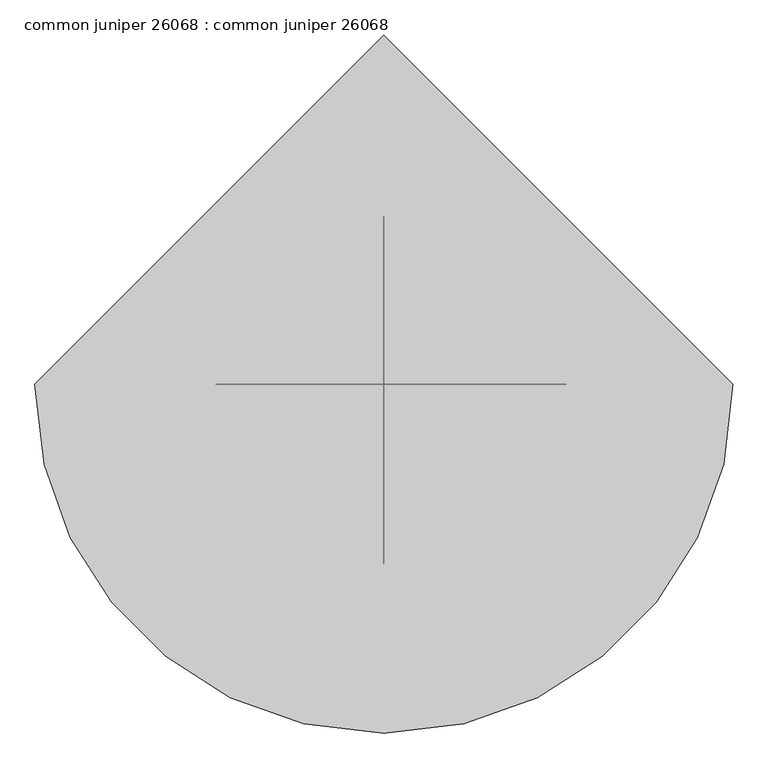
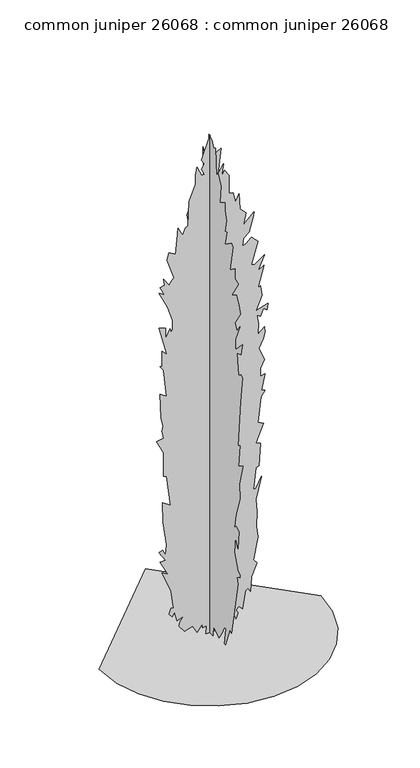
"""IFC4 building model written with IfcOpenShell, lengths in millimetres: proxy geometry, common juniper 26068 : common juniper 26068."""

import ifcopenshell
import ifcopenshell.guid

model = None  # the IFC model being written
_history = None  # IfcOwnerHistory: only IFC2X3 demands one
_inside = {}  # id of a spatial element -> (the spatial element, [elements in it])
_under = {}  # id of a project, library or spatial element -> (it, [spatial elements below it])
_declared = {}  # id of a project -> (the project, [libraries it declares])
_typed = {}  # id of a type object -> (the type object, [elements of that type])
_made_of = {}  # id of a material, layer set ... -> (it, [elements and type objects made of it])


def new_model(schema):
    """Start an empty IFC model of exactly this schema.

    Asked for "IFC4X3", IfcOpenShell would pick the latest addendum, in which some entities
    have other attributes; the version numbers below select the first issue.
    IFC2X3 requires an IfcOwnerHistory on every rooted entity: one is made here for all.
    """
    global model, _history
    if schema == "IFC4X3":
        model = ifcopenshell.file(schema_version=(4, 3, 0, 0))
    else:
        model = ifcopenshell.file(schema=schema)
    _inside.clear()
    _under.clear()
    _declared.clear()
    _typed.clear()
    _made_of.clear()
    _history = None
    if model.schema == "IFC2X3":
        org = make("IfcOrganization", Name="unknown")
        user = make(
            "IfcPersonAndOrganization",
            ThePerson=make("IfcPerson", FamilyName="unknown"),
            TheOrganization=org,
        )
        app = make(
            "IfcApplication",
            ApplicationDeveloper=org,
            Version="unknown",
            ApplicationFullName="unknown",
            ApplicationIdentifier="unknown",
        )
        _history = make(
            "IfcOwnerHistory",
            OwningUser=user,
            OwningApplication=app,
            ChangeAction="ADDED",
            CreationDate=0,
        )
    return model


def make(cls, **values):
    """One entity of the class cls with the attributes given. An attribute that is None is left unset."""
    return model.create_entity(
        cls, **{name: value for name, value in values.items() if value is not None}
    )


def rooted(cls, **values):
    """An entity with a GlobalId (a new one), such as an element, a storey or a relation."""
    return make(cls, GlobalId=ifcopenshell.guid.new(), OwnerHistory=_history, **values)


def si_unit(unit_type, name, prefix=None):
    """IfcSIUnit, for example si_unit("LENGTHUNIT", "METRE", prefix="MILLI")."""
    return make("IfcSIUnit", UnitType=unit_type, Prefix=prefix, Name=name)


def assignment(units):
    """IfcUnitAssignment: the units of a project."""
    return None if units is None else make("IfcUnitAssignment", Units=units)


def point(xyz):
    """IfcCartesianPoint."""
    return None if xyz is None else make("IfcCartesianPoint", Coordinates=xyz)


def direction(xyz):
    """IfcDirection."""
    return None if xyz is None else make("IfcDirection", DirectionRatios=xyz)


def frame(location, z_axis=None, x_axis=None):
    """IfcAxis2Placement3D, a coordinate frame: its origin and axes. An axis left out is left unset."""
    return make(
        "IfcAxis2Placement3D",
        Location=point(location),
        Axis=direction(z_axis),
        RefDirection=direction(x_axis),
    )


def origin():
    """The frame at (0, 0, 0) with its axes left unset."""
    return frame((0.0, 0.0, 0.0))


def place(relative_to, where):
    """IfcLocalPlacement: puts the frame where relative to a parent placement (None: the world)."""
    return make(
        "IfcLocalPlacement", PlacementRelTo=relative_to, RelativePlacement=where
    )


def context(
    kind, dimensions, precision=None, world=None, true_north=None, identifier=None
):
    """IfcGeometricRepresentationContext, for example the 3D "Model" context."""
    return make(
        "IfcGeometricRepresentationContext",
        ContextIdentifier=identifier,
        ContextType=kind,
        CoordinateSpaceDimension=dimensions,
        Precision=precision,
        WorldCoordinateSystem=world,
        TrueNorth=true_north,
    )


def project(units=None, contexts=None):
    """IfcProject with its units and contexts."""
    return rooted(
        "IfcProject",
        Name="project",
        RepresentationContexts=contexts,
        UnitsInContext=assignment(units),
    )


def spatial(cls, under=None, at=None, **own):
    """A site, building, storey or space (cls), placed at a placement, below another one or the project."""
    s = rooted(cls, ObjectPlacement=at, **own)
    if under is not None:
        _under.setdefault(under.id(), (under, []))[1].append(s)
    return s


def point_list(points):
    """IfcCartesianPointList2D or 3D."""
    cls = (
        "IfcCartesianPointList2D" if len(points[0]) == 2 else "IfcCartesianPointList3D"
    )
    return make(cls, CoordList=points)


def triangles(points, corners, closed=None, point_numbers=None):
    """IfcTriangulatedFaceSet: each triangle names its three corners, points numbered from 1."""
    return make(
        "IfcTriangulatedFaceSet",
        Coordinates=point_list(points),
        Closed=closed,
        CoordIndex=corners,
        PnIndex=point_numbers,
    )


def shape(context_of_items, identifier, shape_type, items):
    """IfcShapeRepresentation: the items that make up one representation, for example the "Body"."""
    return make(
        "IfcShapeRepresentation",
        ContextOfItems=context_of_items,
        RepresentationIdentifier=identifier,
        RepresentationType=shape_type,
        Items=items,
    )


def source(mapping_origin, context_of_items, identifier, shape_type, items):
    """IfcRepresentationMap: a shape defined once, which mapped items show again and again."""
    return make(
        "IfcRepresentationMap",
        MappingOrigin=mapping_origin,
        MappedRepresentation=shape(context_of_items, identifier, shape_type, items),
    )


def transform(
    local_origin,
    x_axis=None,
    y_axis=None,
    z_axis=None,
    scale=None,
    scale2=None,
    scale3=None,
    uniform=True,
):
    """IfcCartesianTransformationOperator3D, or its non-uniform kind. x_axis, y_axis, z_axis: its Axis1, 2, 3."""
    if uniform:
        return make(
            "IfcCartesianTransformationOperator3D",
            Axis1=direction(x_axis),
            Axis2=direction(y_axis),
            LocalOrigin=point(local_origin),
            Scale=scale,
            Axis3=direction(z_axis),
        )
    return make(
        "IfcCartesianTransformationOperator3DnonUniform",
        Axis1=direction(x_axis),
        Axis2=direction(y_axis),
        LocalOrigin=point(local_origin),
        Scale=scale,
        Axis3=direction(z_axis),
        Scale2=scale2,
        Scale3=scale3,
    )


def mapped(mapping_source, mapping_target):
    """IfcMappedItem: shows the shape of a source again, moved by a transform."""
    return make(
        "IfcMappedItem", MappingSource=mapping_source, MappingTarget=mapping_target
    )


def made_of(thing, what):
    """Note that an element or type object is made of a material, layer set ...; save() writes the relation."""
    if what is not None:
        _made_of.setdefault(what.id(), (what, []))[1].append(thing)
    return thing


def element(
    cls,
    number,
    at=None,
    inside=None,
    cuts=None,
    type_object=None,
    material=None,
    context=None,
    identifier="Body",
    shape_type=None,
    held_by="IfcProductDefinitionShape",
    body=None,
    shapes=None,
    **own,
):
    """One element of the class cls, such as IfcWall. Its Tag is "e" and its number.

    at: its placement. inside: the storey or other place that contains it. cuts: it is an
    opening in that element (IfcRelVoidsElement). A single representation is given by context,
    identifier, shape_type and body (its items); several are given by shapes. held_by: the class
    of the entity that holds the representations. save() writes the other relations.
    """
    e = rooted(cls, Tag="e%d" % number, ObjectPlacement=at, **own)
    if body is not None:
        shapes = [shape(context, identifier, shape_type, body)]
    if shapes is not None:
        e.Representation = make(held_by, Representations=shapes)
    if inside is not None:
        _inside.setdefault(inside.id(), (inside, []))[1].append(e)
    if cuts is not None:
        rooted(
            "IfcRelVoidsElement", RelatingBuildingElement=cuts, RelatedOpeningElement=e
        )
    if type_object is not None:
        _typed.setdefault(type_object.id(), (type_object, []))[1].append(e)
    return made_of(e, material)


def aggregate(whole, parts):
    """IfcRelAggregates: a whole, such as a stair, and the parts it consists of."""
    return rooted("IfcRelAggregates", RelatingObject=whole, RelatedObjects=parts)


def save(model, path):
    """Write the relations noted so far, then the file.

    IfcRelAggregates (storeys below a building ...), IfcRelContainedInSpatialStructure (elements
    in a storey), IfcRelDefinesByType, IfcRelAssociatesMaterial and IfcRelDeclares: one each for
    every whole, place, type object, material and project.
    """
    for whole, parts in _under.values():
        aggregate(whole, parts)
    for where, things in _inside.values():
        rooted(
            "IfcRelContainedInSpatialStructure",
            RelatedElements=things,
            RelatingStructure=where,
        )
    for kind, things in _typed.values():
        rooted("IfcRelDefinesByType", RelatedObjects=things, RelatingType=kind)
    for what, things in _made_of.values():
        rooted("IfcRelAssociatesMaterial", RelatedObjects=things, RelatingMaterial=what)
    for by, libraries in _declared.values():
        rooted("IfcRelDeclares", RelatingContext=by, RelatedDefinitions=libraries)
    model.write(path)


def common_juniper_26068_common_juniper_26068_35e030ca(model_context):
    return source(origin(), model_context, "Body", "Tessellation", [
        triangles([(2e-06, 20.8572502, 34.4973742), (2.9e-06, 50.3272151, 21.867388), (4.9e-06, 67.1674663, 63.9673119), (4e-06, 75.5873421, 21.867388), (6e-06, 105.0572775, 42.9175021), (6.8e-06, 126.1073371, 38.7074393), (1.05e-05, 163.9974026, 106.0674356), (1.16e-05, 163.9974026, 143.9575011), (1.1e-05, 147.1574058, 148.1673096), (1.26e-05, 147.1574058, 202.8973719), (1.29e-05, 176.6273366, 169.2173783), (1.44e-05, 185.0474622, 207.1074347), (1.33e-05, 155.577277, 211.3174975), (1.5e-05, 155.577277, 270.2568686), (1.59e-05, 172.4172738, 274.4682032), (2.15e-05, 208.9710382, 408.6238226), (2.29e-05, 206.0972674, 459.7084588), (2.67e-05, 248.1971505, 522.8581289), (2.46e-05, 201.8872046, 522.8581289), (2.34e-05, 185.1554134, 508.0702234), (2.48e-05, 172.4172738, 573.376339), (2.87e-05, 210.3073302, 649.1574692), (2.78e-05, 174.6776373, 670.1633818), (3.35e-05, 214.5174112, 800.7172588), (3.23e-05, 197.6771419, 788.0883059), (3.52e-05, 206.0972674, 872.2870182), (4.35e-05, 239.7772792, 1099.6279381), (4.31e-05, 214.5174112, 1124.8883148), (4.64e-05, 221.6324747, 1223.064735), (4.69e-05, 206.0972674, 1263.816608), (5.28e-05, 239.7772792, 1411.1674976), (5.42e-05, 214.5174112, 1495.3662827), (5.6e-05, 239.7772792, 1520.6266594), (5.93e-05, 214.5174112, 1667.977549), (5.58e-05, 162.8142626, 1629.2094212), (5.8e-05, 189.2572706, 1663.7663235), (6.33e-05, 189.2572706, 1840.5863445), (6.26e-05, 176.6273366, 1836.3775898), (6.33e-05, 176.6273366, 1857.4265957), (6.27e-05, 163.9971482, 1857.4265957), (6.42e-05, 172.4172738, 1895.3184689), (6.36e-05, 159.7870854, 1895.3184689), (6.46e-05, 172.4172738, 1907.9474945), (6.6e-05, 184.4045872, 1938.4732475), (6.63e-05, 168.207211, 1971.0971283), (6.38e-05, 138.7372802, 1933.2078712), (6.66e-05, 147.1571514, 2013.1977562), (6.57e-05, 130.3171455, 2008.9863853), (6.57e-05, 113.4776574, 2034.2467621), (6.82e-05, 130.3171455, 2093.1876411), (6.79e-05, 117.6872115, 2101.6077667), (6.74e-05, 115.2719156, 2088.51656), (6.69e-05, 112.8578914, 2076.3093109), (6.65e-05, 110.4461564, 2065.872448), (6.62e-05, 108.0382274, 2058.0897835), (6.59e-05, 105.6348767, 2053.8454205), (6.58e-05, 103.2373577, 2054.0233166), (6.59e-05, 100.8472147, 2059.5071388), (6.74e-05, 67.167212, 2160.5486458), (6.91e-05, 79.797146, 2198.4380482), (6.81e-05, 50.3272151, 2211.0669285), (7.25e-05, 54.7259973, 2350.8028759), (6.92e-05, 29.2771487, 2278.4279331), (6.92e-05, 12.4371758, 2303.6883099), (7e-05, 12.4371758, 2328.9486866), (7.13e-05, 1.9569493, 2388.087664), (7.3e-05, 8.22762, 2438.4078484), (7.15e-05, -17.0328629, 2425.7763519), (7.01e-05, -29.662722, 2396.3072205), (6.96e-05, -46.5027211, 2404.727346), (6.53e-05, -54.9228512, 2274.2165623), (6.54e-05, -63.3427225, 2291.0568134), (6.29e-05, -89.9589621, 2244.0082317), (6.07e-05, -82.3490978, 2159.977169), (5.96e-05, -122.2828521, 2181.597797), (5.84e-05, -122.3656505, 2144.5212811), (5.66e-05, -134.9127861, 2101.6077667), (5.54e-05, -122.2828521, 2042.6668877), (5.48e-05, -138.0380133, 2047.4395615), (5.35e-05, -122.2828521, 1979.5172539), (5.23e-05, -172.8028426, 2013.1977562), (5.13e-05, -186.3878237, 2001.8109512), (4.87e-05, -163.5081882, 1878.2927639), (4.78e-05, -202.2725372, 1907.9474945), (4.63e-05, -202.2725372, 1857.4265957), (4.47e-05, -231.7427224, 1849.0064701), (4.47e-05, -177.0129054, 1764.8078304), (4.36e-05, -214.9027256, 1785.8568363), (4.15e-05, -235.9527852, 1747.9675793), (4e-05, -244.3729108, 1710.0783222), (3.99e-05, -202.2725372, 1642.7171722), (3.83e-05, -219.1127884, 1613.2480408), (3.83e-05, -241.2687761, 1646.3393349), (3.74e-05, -205.5590554, 1563.0676735), (3.58e-05, -206.4828544, 1512.2065338), (3.51e-05, -261.2118902, 1571.1474129), (3.4e-05, -248.5827192, 1512.2065338), (3.5e-05, -219.1127884, 1503.7864082), (3.14e-05, -231.7427224, 1402.7473721), (3.11e-05, -248.5827192, 1415.3763977), (3.03e-05, -261.2118902, 1406.9562721), (2.72e-05, -244.3729108, 1280.6568592), (2.12e-05, -227.5326596, 1053.3184828), (2.09e-05, -240.1625937, 1061.7386084), (1.81e-05, -231.7427224, 956.4883467), (1.73e-05, -265.4232247, 977.5373526), (1.54e-05, -237.9499925, 875.0023321), (1.31e-05, -240.1625937, 800.7172588), (1.16e-05, -210.6926628, 703.8870501), (1.01e-05, -198.0627288, 636.5285889), (9.9e-06, -210.6926628, 649.1574692), (8.4e-06, -235.9527852, 636.5285889), (6.2e-06, -227.5326596, 548.1185057), (8.5e-06, -206.4828544, 594.4279246), (6.5e-06, -198.0627288, 514.4380033), (2.9e-06, -227.5326596, 438.6568731), (2e-06, -243.3599639, 431.2197181), (1.5e-06, -243.5103181, 416.411465), (2.3e-06, -219.1127884, 404.9763708), (1e-06, -227.5326596, 375.5071667), (-4.7e-06, -172.8028426, 101.8573729), (-3.9e-06, -160.1726542, 110.2774984), (-5.1e-06, -126.4926606, 17.6574001), (-4.8e-06, -118.0727893, 17.6574001), (-2.9e-06, -130.7027234, 97.6473101), (-2.4e-06, -118.0727893, 97.6473101), (-2.7e-06, -97.022212, 55.5474361), (-2.7e-06, -71.7625937, 17.6574001), (1e-07, -29.662722, 47.1273105), (-1.2e-06, -26.985301, 2.08e-05), (1.1e-06, 25.0673653, 2.23e-05), (-515.3041569, -1e-07, 3.69e-05), (-501.6820959, -118.0735524, 3.3e-05), (-462.8834467, -226.5052332, 2.86e-05), (-402.0172491, -322.1873471, 2.4e-05), (-322.1873471, -402.0172491, 1.92e-05), (-226.5052332, -462.8834467, 1.45e-05), (-118.0735524, -501.6820959, 1.02e-05), (2.25e-05, -515.3041569, 6.2e-06), (118.0735524, -501.6820959, 3.1e-06), (226.5052332, -462.8834467, 1e-06), (322.1873471, -402.0172491, 0.0), (402.0172491, -322.1873471, 0.0), (462.8834467, -226.5052332, 1e-06), (501.6820959, -118.0735524, 3.1e-06), (515.3041569, 4.49e-05, 6.2e-06), (-6.76e-05, 515.3041569, 3.69e-05), (-18.1277839, 9e-07, 2.21e-05), (-15.9294828, -9e-07, 38.9106382), (-33.6886368, -1e-07, 34.4973742), (-33.6886368, -1.1e-06, 55.5474361), (-58.9485094, 1.2e-06, 21.8674629), (-79.998569, 1e-07, 59.7575034), (-117.8886345, 2.9e-06, 47.1273105), (-143.1485116, 2.2e-06, 80.8073133), (-138.9386941, 0.0, 101.8573729), (-122.098443, -1.5e-06, 122.9074415), (-151.5686372, 0.0, 110.2774984), (-164.1985713, -1.7e-06, 156.5874443), (-176.8285053, -6e-07, 139.7474384), (-189.4584393, -1e-06, 156.5874443), (-181.0385681, -2.3e-06, 181.8473123), (-168.4083797, -2.7e-06, 181.8473123), (-180.3558154, -7.3e-06, 266.0887183), (-223.1384511, -1.18e-05, 371.2983756), (-193.6685021, -1.19e-05, 354.4581244), (-231.5585767, -1.51e-05, 426.0279565), (-206.2984361, -1.59e-05, 426.0279565), (-236.2903554, -1.71e-05, 473.5007129), (-218.928897, -1.91e-05, 480.757501), (-206.2984361, -1.81e-05, 451.2883332), (-202.0883733, -2.05e-05, 501.8065433), (-216.5369645, -2.75e-05, 615.9519379), (-218.928897, -3.28e-05, 712.3071756), (-183.4688521, -3.28e-05, 688.38538), (-202.0883733, -4.12e-05, 838.6065159), (-214.7185799, -4.1e-05, 842.8178867), (-214.7185799, -4.73e-05, 956.4883467), (-248.3983191, -5.04e-05, 1023.8468079), (-214.7185799, -5.16e-05, 1028.058106), (-221.9263521, -5.3e-05, 1065.2057659), (-216.8864708, -5.54e-05, 1088.911659), (-227.3485139, -5.7e-05, 1133.3084404), (-231.5585767, -6.44e-05, 1251.1877277), (-202.0883733, -6.44e-05, 1230.1385765), (-214.7185799, -7.1e-05, 1360.6467442), (-231.5585767, -7.27e-05, 1385.9071209), (-223.1384511, -7.28e-05, 1381.6983662), (-223.1384511, -7.73e-05, 1457.4770256), (-199.0627223, -7.69e-05, 1431.8229229), (-235.7683851, -8.33e-05, 1575.3561676), (-205.5140908, -8.37e-05, 1563.9058491), (-206.2984361, -8.14e-05, 1512.2065338), (-185.2483765, -8.39e-05, 1554.3071617), (-181.0385681, -8.33e-05, 1537.4669106), (-172.6184425, -8.39e-05, 1545.8870361), (-172.4459785, -8.71e-05, 1592.2497585), (-195.9021957, -9.07e-05, 1663.7815842), (-235.7683851, -9.33e-05, 1747.9675793), (-210.5084989, -9.33e-05, 1731.1273281), (-231.5585767, -9.57e-05, 1773.227956), (-210.5084989, -9.65e-05, 1777.4367107), (-214.7185799, -9.77e-05, 1806.9084583), (-189.4584393, -9.68e-05, 1769.0165852), (-176.8285053, -9.92e-05, 1790.0682072), (-165.3669774, -9.99e-05, 1797.7949158), (-197.8783105, -0.0001044, 1895.3184689), (-189.4584393, -0.0001062, 1928.9965004), (-159.9885085, -0.0001063, 1912.1562492), (-151.5683829, -0.0001107, 1979.5172539), (-147.3585744, -0.0001144, 2034.2467621), (-126.3085057, -0.0001131, 1992.1461342), (-113.6788261, -0.000115, 2025.8266365), (-101.0483834, -0.0001167, 2030.0380074), (-96.8383206, -0.0001232, 2147.9172947), (-67.4105474, -0.0001297, 2222.3166779), (-67.3683806, -0.0001316, 2265.7964367), (-58.9482551, -0.0001347, 2303.6883099), (-37.8984453, -0.0001321, 2257.3763111), (-25.268484, -0.0001336, 2257.3763111), (-37.8984453, -0.0001346, 2286.8480587), (-25.268484, -0.0001359, 2307.8970646), (-37.8984453, -0.0001365, 2328.9462158), (-0.0084209, -0.0001447, 2438.4078484), (4.2015544, -0.0001387, 2324.7373158), (21.0416299, -0.0001399, 2341.5775669), (33.6716184, -0.0001405, 2345.786467), (50.5116198, -0.0001427, 2358.4178181), (37.8816812, -0.0001346, 2236.3273052), (63.1415538, -0.0001383, 2278.4279331), (54.7216826, -0.0001341, 2215.2782993), (67.3516166, -0.000137, 2244.7474308), (88.4014264, -0.000135, 2211.0669285), (88.4014264, -0.0001299, 2122.656918), (107.6572278, -0.0001303, 2118.4099388), (117.8716207, -0.0001285, 2072.1386353), (134.7116175, -0.0001316, 2105.8166668), (138.9216803, -0.0001272, 2030.0380074), (168.3916111, -0.0001268, 2000.5662598), (155.7614227, -0.0001229, 1945.8367516), (205.6238225, -0.0001275, 1992.2782482), (202.8546965, -0.0001267, 1974.4448891), (182.6657035, -0.0001205, 1900.3248493), (155.7614227, -0.0001187, 1878.4782177), (151.5516143, -0.000116, 1844.7977154), (168.3916111, -0.0001178, 1849.0064701), (193.6514973, -0.0001195, 1870.0580921), (223.1216825, -0.000119, 1840.5863445), (193.6514973, -0.0001114, 1739.5474537), (206.2816857, -0.0001114, 1731.1273281), (252.5916133, -0.0001165, 1764.8078304), (223.1216825, -0.0001104, 1697.4468258), (251.7186107, -0.000113, 1712.8392002), (223.1216825, -0.0001055, 1613.2480408), (235.7516165, -0.000106, 1617.4567955), (242.5560522, -0.0001041, 1569.0011776), (214.7015569, -9.92e-05, 1503.7864082), (269.4313558, -0.0001027, 1520.6266594), (265.2225647, -0.0001001, 1491.1575279), (248.3815506, -0.0001002, 1503.7864082), (235.7516165, -9.72e-05, 1470.1083767), (218.9116197, -9.71e-05, 1478.5285023), (225.9123915, -9.55e-05, 1438.523386), (223.1214282, -9.19e-05, 1385.9071209), (252.5916133, -9.51e-05, 1411.1674976), (256.8024392, -9.41e-05, 1385.9071209), (248.3815506, -9.14e-05, 1356.4379894), (227.3314909, -8.77e-05, 1314.3373615), (252.5916133, -8.56e-05, 1251.1877277), (235.7516165, -8.23e-05, 1213.298398), (235.7516165, -8.06e-05, 1175.4065248), (256.8024392, -8.14e-05, 1179.6178957), (239.961425, -7.64e-05, 1103.8367655), (256.8024392, -7.67e-05, 1099.6279381), (237.7775285, -7.39e-05, 1074.3497572), (223.1214282, -6.58e-05, 952.2769758), (248.3815506, -6.71e-05, 939.6480955), (214.7015569, -6.01e-05, 855.446767), (235.7513622, -6.03e-05, 847.0266415), (227.3314909, -5.4e-05, 737.5675524), (214.7015569, -5.23e-05, 733.3562542), (202.0711142, -4.63e-05, 632.317218), (214.7015569, -4.67e-05, 632.317218), (239.961425, -5.08e-05, 682.8379715), (214.7015569, -4.31e-05, 577.5876735), (218.9116197, -4.06e-05, 518.6467944), (216.6522736, -3.6e-05, 443.0028288), (223.1214282, -3.28e-05, 392.3474178), (202.0711142, -2.52e-05, 287.0971198), (218.9116197, -2.48e-05, 266.0480776), (193.6514973, -2.03e-05, 207.1074347), (189.4414345, -1.58e-05, 135.5373756), (176.8114823, -1.64e-05, 156.5874443), (164.1815483, -1.56e-05, 148.1673096), (151.5513599, -1.04e-05, 63.9673119), (134.7116175, -1.06e-05, 80.8073133), (122.0814291, -9.7e-06, 68.1773747), (130.5015547, -8e-06, 51.3373733), (122.0814291, -6.7e-06, 26.0775007), (113.6615579, -7.2e-06, 42.9172477), (75.7714924, -5.9e-06, 38.7074393), (71.561425, -3.1e-06, 5.0273616), (63.1415538, -3.8e-06, 26.0775007), (50.5113654, -4e-06, 38.7074393), (16.5476705, -2.2e-06, 20.6906271), (21.2391151, -2e-07, 2.1e-05)], [[92, 93, 94], [61, 62, 63], [112, 113, 114], [95, 96, 97], [95, 97, 98], [23, 24, 25], [105, 106, 107], [103, 104, 105], [83, 84, 85], [10, 11, 12], [10, 12, 13], [71, 72, 73], [17, 18, 19], [17, 19, 20], [66, 67, 68], [66, 68, 69], [78, 79, 80], [74, 75, 76], [33, 34, 35], [44, 45, 46], [43, 44, 46], [3, 4, 5], [50, 51, 52], [49, 50, 52], [49, 52, 53], [49, 53, 54], [49, 54, 55], [49, 55, 56], [69, 70, 71], [120, 121, 122], [46, 47, 48], [36, 37, 38], [85, 86, 87], [40, 41, 42], [123, 124, 125], [122, 123, 125], [111, 112, 114], [110, 111, 114], [42, 43, 46], [130, 131, 1], [129, 130, 1], [66, 69, 71], [65, 66, 71], [64, 65, 71], [1, 2, 3], [127, 128, 129], [87, 88, 89], [38, 39, 40], [21, 22, 23], [59, 60, 61], [32, 33, 35], [63, 64, 71], [83, 85, 87], [7, 8, 9], [61, 63, 71], [80, 81, 82], [80, 82, 83], [5, 6, 7], [3, 5, 7], [3, 7, 9], [61, 71, 73], [61, 73, 74], [59, 61, 74], [58, 59, 74], [99, 100, 101], [99, 101, 102], [117, 118, 119], [116, 117, 119], [49, 56, 57], [87, 89, 90], [87, 90, 91], [14, 15, 16], [126, 127, 129], [26, 27, 28], [74, 76, 77], [58, 74, 77], [58, 77, 78], [58, 78, 80], [57, 58, 80], [49, 57, 80], [48, 49, 80], [46, 48, 80], [46, 80, 83], [46, 83, 87], [42, 46, 87], [40, 42, 87], [38, 40, 87], [36, 38, 87], [35, 36, 87], [35, 87, 91], [32, 35, 91], [32, 91, 92], [32, 92, 94], [32, 94, 95], [31, 32, 95], [30, 31, 95], [30, 95, 98], [30, 98, 99], [30, 99, 102], [30, 102, 103], [29, 30, 103], [28, 29, 103], [26, 28, 103], [26, 103, 105], [26, 105, 107], [25, 26, 107], [25, 107, 108], [25, 108, 109], [23, 25, 109], [23, 109, 110], [21, 23, 110], [21, 110, 114], [21, 114, 115], [20, 21, 115], [20, 115, 116], [20, 116, 119], [17, 20, 119], [16, 17, 119], [14, 16, 119], [14, 119, 120], [14, 120, 122], [14, 122, 125], [14, 125, 126], [13, 14, 126], [10, 13, 126], [10, 126, 129], [9, 10, 129], [3, 9, 129], [1, 3, 129], [146, 147, 132], [145, 146, 132], [145, 132, 133], [144, 145, 133], [144, 133, 134], [144, 134, 135], [143, 144, 135], [142, 143, 135], [142, 135, 136], [142, 136, 137], [142, 137, 138], [142, 138, 139], [142, 139, 140], [142, 140, 141], [283, 284, 285], [223, 224, 225], [229, 230, 231], [202, 203, 204], [301, 302, 303], [236, 237, 238], [186, 187, 188], [250, 251, 252], [210, 211, 212], [198, 199, 200], [291, 292, 293], [217, 218, 219], [164, 165, 166], [240, 241, 242], [193, 194, 195], [188, 189, 190], [240, 242, 243], [298, 299, 300], [252, 253, 254], [227, 228, 229], [183, 184, 185], [222, 223, 225], [294, 295, 296], [173, 174, 175], [231, 232, 233], [264, 265, 266], [258, 259, 260], [257, 258, 260], [166, 167, 168], [151, 152, 153], [271, 272, 273], [273, 274, 275], [257, 260, 261], [257, 261, 262], [178, 179, 180], [159, 160, 161], [159, 161, 162], [159, 162, 163], [226, 227, 229], [225, 226, 229], [264, 266, 267], [216, 217, 219], [207, 208, 209], [200, 201, 202], [200, 202, 204], [149, 150, 151], [305, 306, 148], [305, 148, 149], [254, 255, 256], [168, 169, 170], [168, 170, 171], [222, 225, 229], [221, 222, 229], [220, 221, 229], [157, 158, 159], [297, 298, 300], [282, 283, 285], [301, 303, 304], [276, 277, 278], [246, 247, 248], [246, 248, 249], [245, 246, 249], [206, 207, 209], [231, 233, 234], [240, 243, 244], [278, 279, 280], [278, 280, 281], [153, 154, 155], [153, 155, 156], [153, 156, 157], [176, 177, 178], [191, 192, 193], [190, 191, 193], [264, 267, 268], [297, 300, 301], [234, 235, 236], [289, 290, 291], [238, 239, 240], [304, 305, 149], [209, 210, 212], [151, 153, 157], [212, 213, 214], [190, 193, 195], [216, 219, 220], [216, 220, 229], [215, 216, 229], [215, 229, 231], [215, 231, 234], [214, 215, 234], [214, 234, 236], [214, 236, 238], [214, 238, 240], [212, 214, 240], [212, 240, 244], [209, 212, 244], [206, 209, 244], [206, 244, 245], [206, 245, 249], [186, 188, 190], [254, 256, 257], [268, 269, 270], [205, 206, 249], [204, 205, 249], [200, 204, 249], [198, 200, 249], [197, 198, 249], [196, 197, 249], [196, 249, 250], [196, 250, 252], [196, 252, 254], [196, 254, 257], [196, 257, 262], [196, 262, 263], [196, 263, 264], [195, 196, 264], [190, 195, 264], [186, 190, 264], [185, 186, 264], [185, 264, 268], [185, 268, 270], [185, 270, 271], [183, 185, 271], [182, 183, 271], [182, 271, 273], [182, 273, 275], [182, 275, 276], [181, 182, 276], [180, 181, 276], [178, 180, 276], [176, 178, 276], [176, 276, 278], [175, 176, 278], [175, 278, 281], [175, 281, 282], [173, 175, 282], [172, 173, 282], [172, 282, 285], [172, 285, 286], [172, 286, 287], [171, 172, 287], [168, 171, 287], [166, 168, 287], [166, 287, 288], [166, 288, 289], [164, 166, 289], [164, 289, 291], [163, 164, 291], [163, 291, 293], [163, 293, 294], [163, 294, 296], [159, 163, 296], [157, 159, 296], [151, 157, 296], [151, 296, 297], [151, 297, 301], [151, 301, 304], [151, 304, 149]], closed=False),
    ])


if __name__ == "__main__":
    model = new_model("IFC4")
    model_context = context("Model", 3, world=origin())
    ifc_project = project(units=[si_unit("LENGTHUNIT", "METRE", prefix="MILLI")], contexts=[model_context])
    site = spatial("IfcSite", under=ifc_project)
    building = spatial("IfcBuilding", under=site)
    placement = place(None, origin())
    common_juniper_26068_common_juniper_26068_shape = common_juniper_26068_common_juniper_26068_35e030ca(model_context)
    element("IfcBuildingElementProxy", 1, Name="common juniper 26068 : common juniper 26068", ObjectType="common juniper 26068 : common juniper 26068", at=placement, inside=building, context=model_context, shape_type="MappedRepresentation", body=[
        mapped(common_juniper_26068_common_juniper_26068_shape, transform((0.0, 0.0, 0.0), x_axis=(1.0, 0.0, 0.0), y_axis=(0.0, 1.0, 0.0), z_axis=(0.0, 0.0, 1.0))),
    ])
    save(model, "model.ifc")

# Revit data of these elements
# Type "common juniper 26068 : common juniper 26068"
#   built-in parameter 1005195 = "RPC-16-G3GW-Q1G0-PMP1-8000-ST1L-LVER-AU"
#   Height = 0
